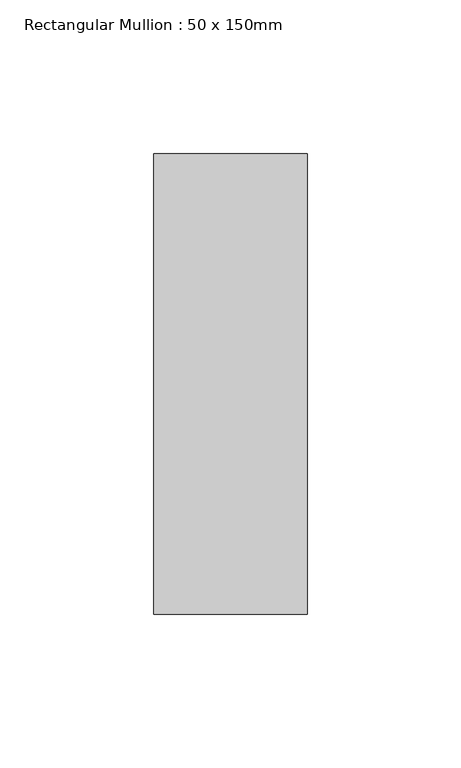
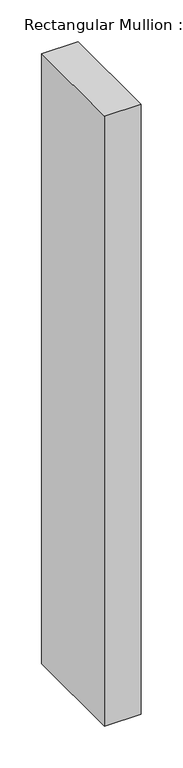
"""IFC4 building model written with IfcOpenShell, lengths in millimetres: member geometry, Rectangular Mullion : 50 x 150mm."""

from ifc_helpers import new_model, si_unit, frame, origin, place, context, project, spatial, polyline, outline, extrude, source, transform, mapped, element, save


def rectangular_mullion_50_x_150mm_8ee200a5(model_context):
    return source(origin(), model_context, "Body", "SweptSolid", [
        extrude(outline(polyline([(0.0, 75.0), (0.0, -75.0), (-50.0, -75.0), (-50.0, 75.0), (0.0, 75.0)])), frame((0.0, 0.0, -887.5), z_axis=(0.0, 0.0, 1.0), x_axis=(1.0, 0.0, 0.0)), (0.0, 0.0, 1.0), 887.5),
    ])


if __name__ == "__main__":
    model = new_model("IFC4")
    model_context = context("Model", 3, world=origin())
    ifc_project = project(units=[si_unit("LENGTHUNIT", "METRE", prefix="MILLI")], contexts=[model_context])
    site = spatial("IfcSite", under=ifc_project)
    building = spatial("IfcBuilding", under=site)
    placement = place(None, origin())
    rectangular_mullion_50_x_150mm_shape = rectangular_mullion_50_x_150mm_8ee200a5(model_context)
    element("IfcMember", 1, ObjectType="Rectangular Mullion : 50 x 150mm", at=placement, inside=building, context=model_context, shape_type="MappedRepresentation", body=[
        mapped(rectangular_mullion_50_x_150mm_shape, transform((0.0, 0.0, 0.0), x_axis=(1.0, 0.0, 0.0), y_axis=(0.0, 1.0, 0.0), z_axis=(0.0, 0.0, 1.0))),
    ])
    save(model, "model.ifc")

# Revit data of these elements
# Type "Rectangular Mullion : 50 x 150mm"
#   built-in parameter 1007304 = 0.492126 (stored number, unit not read)
#   built-in parameter 1007301 = 0.082021 (stored number, unit not read)
#   built-in parameter 1007300 = 0.082021 (stored number, unit not read)
# Element 1 (IfcMember, "Rectangular Mullion : 50 x 150mm")
#   Materials on its faces: "Aluminium"
# Materials
#   "Aluminium": class "Metal", colour RGB 247 247 247, transparency 0, Description = "Aluminium 6061", Cost = 0
